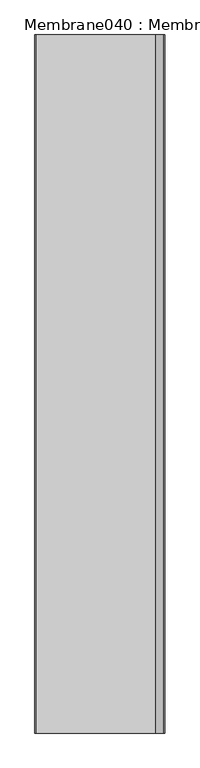
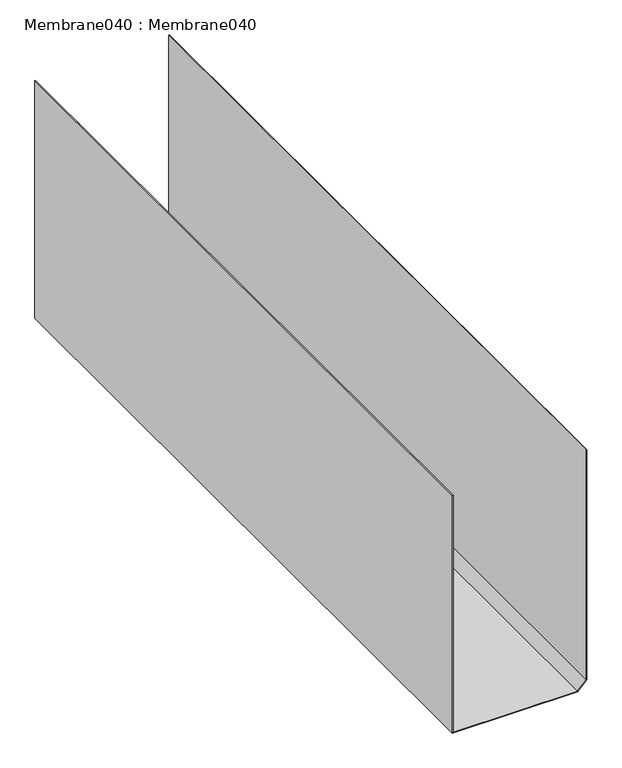
"""IFC4 building model written with IfcOpenShell, lengths in millimetres: proxy geometry, Membrane040 : Membrane040."""

from ifc_helpers import new_model, si_unit, frame, origin, place, context, project, spatial, polyline, outline, extrude, source, transform, mapped, element, save


def membrane040_membrane040_042d28cd(model_context):
    return source(origin(), model_context, "Body", "SweptSolid", [
        extrude(outline(polyline([(33312.9960937, -9692.7802734), (32641.4980103, -9692.7802734), (32616.7480469, -9716.9438184), (32616.7480469, -10060.5869141), (33309.0146212, -10060.5869141), (33309.0146212, -10062.5869141), (32614.7480469, -10062.5869141), (32614.7480469, -9716.101311), (32640.6835937, -9690.7802734), (33312.9960937, -9690.7802734), (33312.9960937, -9692.7802734)])), frame((0.0, 7982.1531721, 0.0), z_axis=(0.0, 1.0, 0.0), x_axis=(0.0, 0.0, 1.0)), (0.0, 0.0, 1.0), 2000.0),
    ])


if __name__ == "__main__":
    model = new_model("IFC4")
    model_context = context("Model", 3, world=origin())
    ifc_project = project(units=[si_unit("LENGTHUNIT", "METRE", prefix="MILLI")], contexts=[model_context])
    site = spatial("IfcSite", under=ifc_project)
    building = spatial("IfcBuilding", under=site)
    placement = place(None, origin())
    membrane040_membrane040_shape = membrane040_membrane040_042d28cd(model_context)
    element("IfcBuildingElementProxy", 1, Name="Membrane040 : Membrane040", ObjectType="Membrane040 : Membrane040", at=placement, inside=building, context=model_context, shape_type="MappedRepresentation", body=[
        mapped(membrane040_membrane040_shape, transform((0.0, 0.0, 0.0), x_axis=(1.0, 0.0, 0.0), y_axis=(0.0, 1.0, 0.0), z_axis=(0.0, 0.0, 1.0))),
    ])
    save(model, "model.ifc")

# Revit data of these elements
# Type "Membrane040 : Membrane040"
#   NameOverride = "Membrane040"
# Element 1 (IfcBuildingElementProxy, "Membrane040 : Membrane040")
#   Materials on its faces: "GEOTEXTILE FILTER FABRIC"
# Materials
#   "GEOTEXTILE FILTER FABRIC": class "Unassigned", colour RGB 254 255 135, transparency 0
